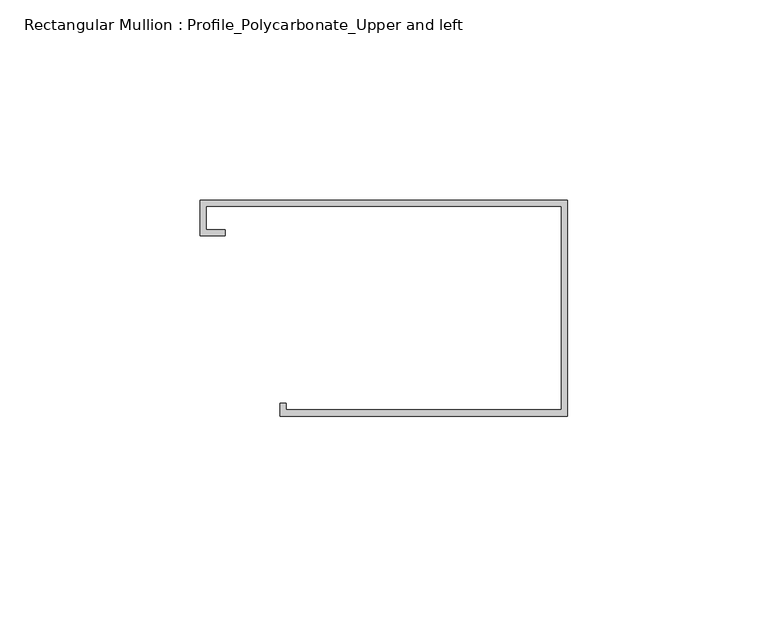
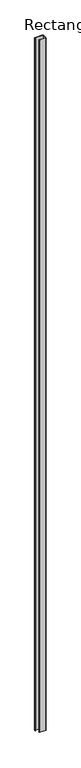
"""IFC4 building model written with IfcOpenShell, lengths in millimetres: member geometry, Rectangular Mullion : Profile_Polycarbonate_Upper and left."""

from ifc_helpers import new_model, si_unit, frame, origin, place, context, project, spatial, polyline, outline, extrude, source, transform, mapped, element, save


def rectangular_mullion_profile_polycarbonate_upper_and_left_a906cc12(model_context):
    return source(origin(), model_context, "Body", "SweptSolid", [
        extrude(outline(polyline([(0.0, 28.984575), (0.0, -25.015825), (-71.9836, -25.015825), (-71.9836, -21.840825), (-70.3961, -21.840825), (-70.3961, -23.428325), (-1.5875, -23.428325), (-1.5875, 27.397075), (-90.4113, 27.397075), (-90.4113, 21.580475), (-85.6488, 21.580475), (-85.6488, 19.992975), (-91.9988, 19.992975), (-91.9988, 28.984575), (0.0, 28.984575)])), frame((0.0, 0.0, -7918.6024), z_axis=(0.0, 0.0, 1.0), x_axis=(1.0, 0.0, 0.0)), (0.0, 0.0, 1.0), 7918.6024),
    ])


if __name__ == "__main__":
    model = new_model("IFC4")
    model_context = context("Model", 3, world=origin())
    ifc_project = project(units=[si_unit("LENGTHUNIT", "METRE", prefix="MILLI")], contexts=[model_context])
    site = spatial("IfcSite", under=ifc_project)
    building = spatial("IfcBuilding", under=site)
    placement = place(None, origin())
    rectangular_mullion_profile_polycarbonate_upper_and_left_shape = rectangular_mullion_profile_polycarbonate_upper_and_left_a906cc12(model_context)
    element("IfcMember", 1, ObjectType="Rectangular Mullion : Profile_Polycarbonate_Upper and left", at=placement, inside=building, context=model_context, shape_type="MappedRepresentation", body=[
        mapped(rectangular_mullion_profile_polycarbonate_upper_and_left_shape, transform((0.0, 0.0, 0.0), x_axis=(1.0, 0.0, 0.0), y_axis=(0.0, 1.0, 0.0), z_axis=(0.0, 0.0, 1.0))),
    ])
    save(model, "model.ifc")

# Revit data of these elements
# Type "Rectangular Mullion : Profile_Polycarbonate_Upper and left"
#   built-in parameter 1007322 = 0.177167 (stored number, unit not read)
#   built-in parameter 1007321 = 0.00520833 (stored number, unit not read)
#   built-in parameter 1007320 = 0 (stored number, unit not read)
